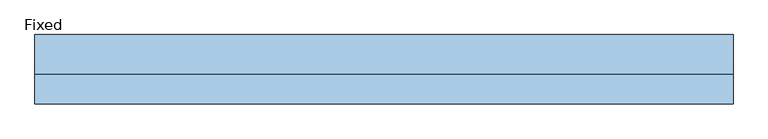
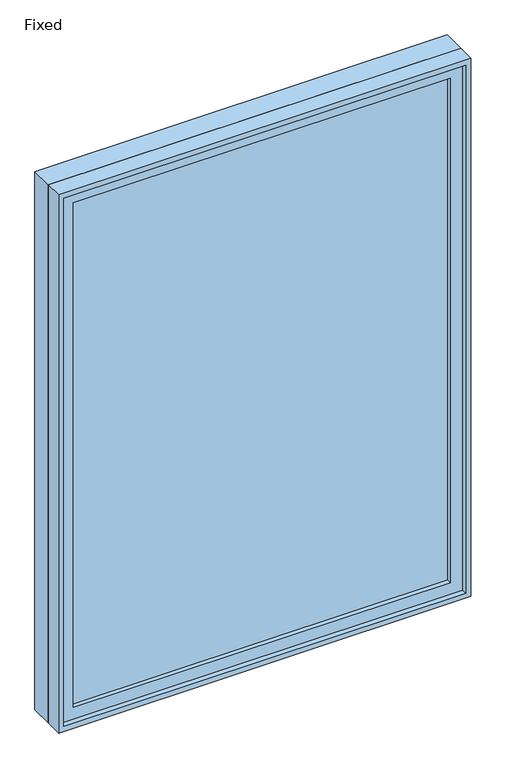
"""IFC4 building model written with IfcOpenShell, lengths in millimetres: window geometry, Fixed."""

from ifc_helpers import new_model, si_unit, frame, origin, place, context, project, spatial, polyline, outline, extrude, source, transform, mapped, element, save


def fixed_94d97772(model_context):
    return source(origin(), model_context, "Body", "SweptSolid", [
        extrude(outline(polyline([(635.0, -25.4), (635.0, -38.1), (-711.2, -38.1), (-711.2, -25.4), (635.0, -25.4)])), frame((0.0, 0.0, 977.9), z_axis=(0.0, 0.0, 1.0), x_axis=(1.0, 0.0, 0.0)), (0.0, 0.0, 1.0), 1905.0),
        extrude(outline(polyline([(2927.35, -755.65), (933.45, -755.65), (933.45, 679.45), (2927.35, 679.45), (2927.35, -755.65)]), holes=[polyline([(2882.9, -711.2), (2882.9, 635.0), (977.9, 635.0), (977.9, -711.2), (2882.9, -711.2)])]), frame((0.0, -53.975, 0.0), z_axis=(0.0, 1.0, 0.0), x_axis=(0.0, 0.0, 1.0)), (0.0, 0.0, 1.0), 44.45),
        extrude(outline(polyline([(2946.4, -774.7), (914.4, -774.7), (914.4, 698.5), (2946.4, 698.5), (2946.4, -774.7)]), holes=[polyline([(2914.65, -742.95), (2914.65, 666.75), (946.15, 666.75), (946.15, -742.95), (2914.65, -742.95)])]), frame((0.0, -9.525, 0.0), z_axis=(0.0, 1.0, 0.0), x_axis=(0.0, 0.0, 1.0)), (0.0, 0.0, 1.0), 82.55),
        extrude(outline(polyline([(2946.4, 698.5), (2946.4, -774.7), (914.4, -774.7), (914.4, 698.5), (2946.4, 698.5)]), holes=[polyline([(2927.35, 679.45), (933.45, 679.45), (933.45, -755.65), (2927.35, -755.65), (2927.35, 679.45)])]), frame((0.0, -73.025, 0.0), z_axis=(0.0, 1.0, 0.0), x_axis=(0.0, 0.0, 1.0)), (0.0, 0.0, 1.0), 63.5),
    ])


if __name__ == "__main__":
    model = new_model("IFC4")
    model_context = context("Model", 3, world=origin())
    ifc_project = project(units=[si_unit("LENGTHUNIT", "METRE", prefix="MILLI")], contexts=[model_context])
    site = spatial("IfcSite", under=ifc_project)
    building = spatial("IfcBuilding", under=site)
    placement = place(None, origin())
    fixed_shape = fixed_94d97772(model_context)
    element("IfcWindow", 1, ObjectType="Fixed : 58\"x80\"@11\"", at=placement, inside=building, context=model_context, shape_type="MappedRepresentation", body=[
        mapped(fixed_shape, transform((0.0, 0.0, 0.0), x_axis=(1.0, 0.0, 0.0), y_axis=(0.0, 1.0, 0.0), z_axis=(0.0, 0.0, 1.0))),
    ])
    save(model, "model.ifc")

# Revit data of these elements
# Type "Fixed : 58\"x80\"@11\""
#   Type Mark = "19"
#   Construction Type Id = "GSP4R"
#   Assembly Code = "B2020100"
#   Analytic Construction = "1/8 in Pilkington single glazing"
#   Visual Light Transmittance = 0.9
#   Solar Heat Gain Coefficient = 0.78
#   Heat Transfer Coefficient (U) = 3.6886 W/(m²·K)
#   Height = 6' - 8"
#   Default Sill Height = 3' - 0"
#   Width = 4' - 10"
#   Window Inset = 0' - 0 3/4"
#   Glass Pane Material = Glass
#   Sash Material = Metal Trim
#   Wall Closure = (empty or 0)
# Element 1 (IfcWindow, "Fixed : 58\"x80\"@11\"")
#   Materials on its faces: "Metal Trim", "Glass"
# Materials
#   "Glass": class "Glass", colour RGB 218 227 224, transparency 0.85, Description = "Soda Lime Glass", Cost = 0
#   "Metal Trim": class "Wood", colour RGB 151 137 121, transparency 0, Cost = 0
